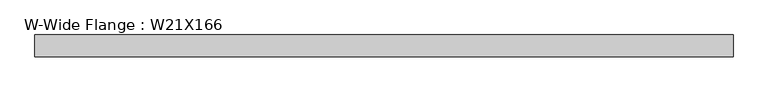
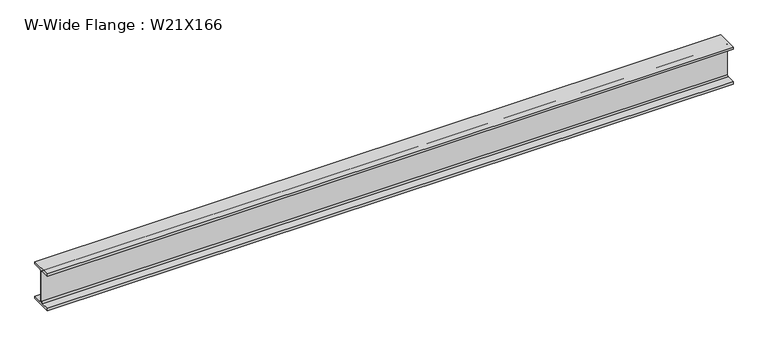
"""IFC4 building model written with IfcOpenShell, lengths in millimetres: beam geometry, W-Wide Flange : W21X166."""

from ifc_helpers import new_model, si_unit, point, frame, frame_2d, origin, place, context, project, spatial, polyline, circle_curve, trimmed, segment, composite_curve, outline, extrude, source, transform, mapped, element, save


def w_wide_flange_w21x166_98a64792(model_context):
    return source(origin(), model_context, "Body", "SweptSolid", [
        extrude(outline(composite_curve([segment(polyline([(157.48, -251.206), (157.48, -285.75), (-157.48, -285.75), (-157.48, -251.206), (-32.131, -251.206)]), True, "CONTINUOUS"), segment(trimmed(circle_curve(frame_2d((-32.131, -228.6)), 22.606), [point((-32.131, -251.206))], [point((-9.525, -228.6))], True, "CARTESIAN"), True, "CONTINUOUS"), segment(polyline([(-9.525, -228.6), (-9.525, 228.6)]), True, "CONTINUOUS"), segment(trimmed(circle_curve(frame_2d((-32.131, 228.6)), 22.606), [point((-9.525, 228.6))], [point((-32.131, 251.206))], True, "CARTESIAN"), True, "CONTINUOUS"), segment(polyline([(-32.131, 251.206), (-157.48, 251.206), (-157.48, 285.75), (157.48, 285.75), (157.48, 251.206), (32.131, 251.206)]), True, "CONTINUOUS"), segment(trimmed(circle_curve(frame_2d((32.131, 228.6)), 22.606), [point((32.131, 251.206))], [point((9.525, 228.6))], True, "CARTESIAN"), True, "CONTINUOUS"), segment(polyline([(9.525, 228.6), (9.525, -228.6)]), True, "CONTINUOUS"), segment(trimmed(circle_curve(frame_2d((32.131, -228.6)), 22.606), [point((9.525, -228.6))], [point((32.131, -251.206))], True, "CARTESIAN"), True, "CONTINUOUS"), segment(polyline([(32.131, -251.206), (157.48, -251.206)]), True, "CONTINUOUS")], self_intersect=False)), frame((-4963.0833357, 0.0, 0.0), z_axis=(1.0, 0.0, 0.0), x_axis=(0.0, 1.0, 0.0)), (0.0, 0.0, 1.0), 10061.6548886),
    ])


if __name__ == "__main__":
    model = new_model("IFC4")
    model_context = context("Model", 3, world=origin())
    ifc_project = project(units=[si_unit("LENGTHUNIT", "METRE", prefix="MILLI")], contexts=[model_context])
    site = spatial("IfcSite", under=ifc_project)
    building = spatial("IfcBuilding", under=site)
    placement = place(None, origin())
    w_wide_flange_w21x166_shape = w_wide_flange_w21x166_98a64792(model_context)
    element("IfcBeam", 1, ObjectType="W-Wide Flange : W21X166", at=placement, inside=building, context=model_context, shape_type="MappedRepresentation", body=[
        mapped(w_wide_flange_w21x166_shape, transform((0.0, 0.0, 0.0), x_axis=(1.0, 0.0, 0.0), y_axis=(0.0, 1.0, 0.0), z_axis=(0.0, 0.0, 1.0))),
    ])
    save(model, "model.ifc")

# Revit data of these elements
# Type "W-Wide Flange : W21X166"
#   Assembly Code = "B10"
#   W = 166
#   Length [instance default] = 5' - 0"
#   bf = 1' - 0.4"
#   d = 1' - 10 1/2"
#   k = 0' - 2 1/4"
#   k2 = 0' - 0.89"
#   tf = 0' - 1.36"
#   tw = 0' - 0 3/4"
#   A = 0.338889 SF
#   Structural Material [instance default] = Steel ASTM A992
# Element 1 (IfcBeam, "W-Wide Flange : W21X166")
#   Materials on its faces: "Steel ASTM A992"
# Materials
#   "Steel ASTM A992": class "Metal", colour RGB 199 199 199, transparency 0, Description = "Structural steel 50ksi", Cost = 0
